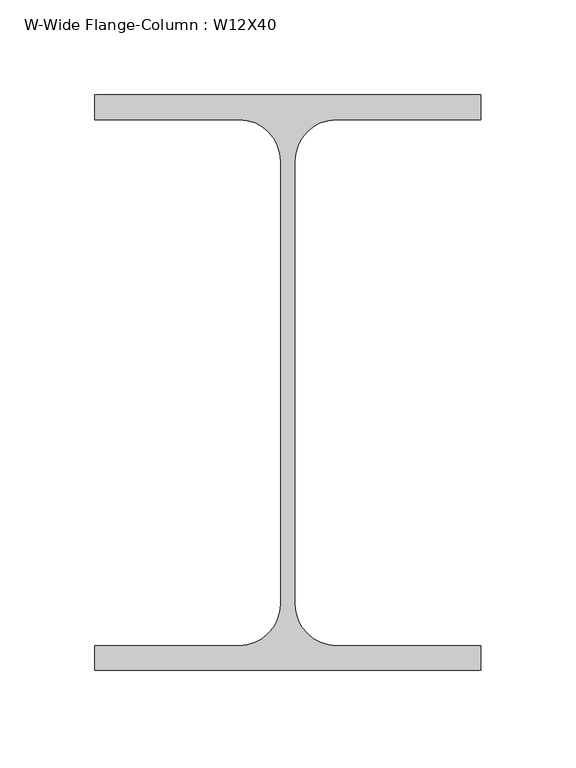
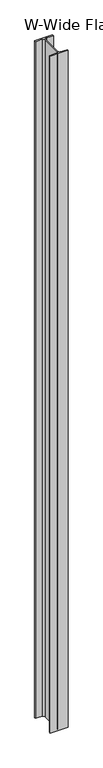
"""IFC4 building model written with IfcOpenShell, lengths in millimetres: column geometry, W-Wide Flange-Column : W12X40."""

from ifc_helpers import new_model, si_unit, point, frame, frame_2d, origin, place, context, project, spatial, polyline, circle_curve, trimmed, segment, composite_curve, outline, extrude, source, transform, mapped, element, save


def w_wide_flange_column_w12x40_d1cfc84d(model_context):
    return source(origin(), model_context, "Body", "SweptSolid", [
        extrude(outline(composite_curve([segment(polyline([(101.6496094, 151.6558594), (101.6496094, 138.5589844), (25.5984375, 138.5589844)]), True, "CONTINUOUS"), segment(trimmed(circle_curve(frame_2d((25.5984375, 116.7308594)), 21.828125), [point((25.5984375, 138.5589844))], [point((3.7703125, 116.7308594))], True, "CARTESIAN"), True, "CONTINUOUS"), segment(polyline([(3.7703125, 116.7308594), (3.7703125, -116.7308594)]), True, "CONTINUOUS"), segment(trimmed(circle_curve(frame_2d((25.5984375, -116.7308594)), 21.828125), [point((3.7703125, -116.7308594))], [point((25.5984375, -138.5589844))], True, "CARTESIAN"), True, "CONTINUOUS"), segment(polyline([(25.5984375, -138.5589844), (101.6496094, -138.5589844), (101.6496094, -151.6558594), (-101.6496094, -151.6558594), (-101.6496094, -138.5589844), (-25.5984375, -138.5589844)]), True, "CONTINUOUS"), segment(trimmed(circle_curve(frame_2d((-25.5984375, -116.7308594)), 21.828125), [point((-25.5984375, -138.5589844))], [point((-3.7703125, -116.7308594))], True, "CARTESIAN"), True, "CONTINUOUS"), segment(polyline([(-3.7703125, -116.7308594), (-3.7703125, 116.7308594)]), True, "CONTINUOUS"), segment(trimmed(circle_curve(frame_2d((-25.5984375, 116.7308594)), 21.828125), [point((-3.7703125, 116.7308594))], [point((-25.5984375, 138.5589844))], True, "CARTESIAN"), True, "CONTINUOUS"), segment(polyline([(-25.5984375, 138.5589844), (-101.6496094, 138.5589844), (-101.6496094, 151.6558594), (101.6496094, 151.6558594)]), True, "CONTINUOUS")], self_intersect=False)), frame((0.0, 0.0, 30302.2), z_axis=(0.0, 0.0, 1.0), x_axis=(1.0, 0.0, 0.0)), (0.0, 0.0, 1.0), 8102.6),
    ])


if __name__ == "__main__":
    model = new_model("IFC4")
    model_context = context("Model", 3, world=origin())
    ifc_project = project(units=[si_unit("LENGTHUNIT", "METRE", prefix="MILLI")], contexts=[model_context])
    site = spatial("IfcSite", under=ifc_project)
    building = spatial("IfcBuilding", under=site)
    placement = place(None, origin())
    w_wide_flange_column_w12x40_shape = w_wide_flange_column_w12x40_d1cfc84d(model_context)
    element("IfcColumn", 1, ObjectType="W-Wide Flange-Column : W12X40", at=placement, inside=building, context=model_context, shape_type="MappedRepresentation", body=[
        mapped(w_wide_flange_column_w12x40_shape, transform((0.0, 0.0, 0.0), x_axis=(1.0, 0.0, 0.0), y_axis=(0.0, 1.0, 0.0), z_axis=(0.0, 0.0, 1.0))),
    ])
    save(model, "model.ifc")

# Revit data of these elements
# Type "W-Wide Flange-Column : W12X40"
#   Assembly Code = "B10"
#   W = 40
#   bf = 203.299 mm
#   d = 303.312 mm
#   k = 34.925 mm
#   kr = 21.828 mm
#   tf = 13.097 mm
#   tw = 7.541 mm
#   A = 0.00761289 m²
#   Structural Material [instance default] = Steel ASTM A992
# Element 1 (IfcColumn, "W-Wide Flange-Column : W12X40")
#   Structural Material = Aluminum, Anodized Red
#   Materials on its faces: "Aluminum, Anodized Red"
# Materials
#   "Steel ASTM A992": class "Metal", colour RGB 128 0 0, transparency 0, Description = "Structural steel 50ksi", Cost = 0
#   "Aluminum, Anodized Red": class "Metal", colour RGB 120 120 120, transparency 0, Description = "Anodized aluminum, red", Cost = 0
